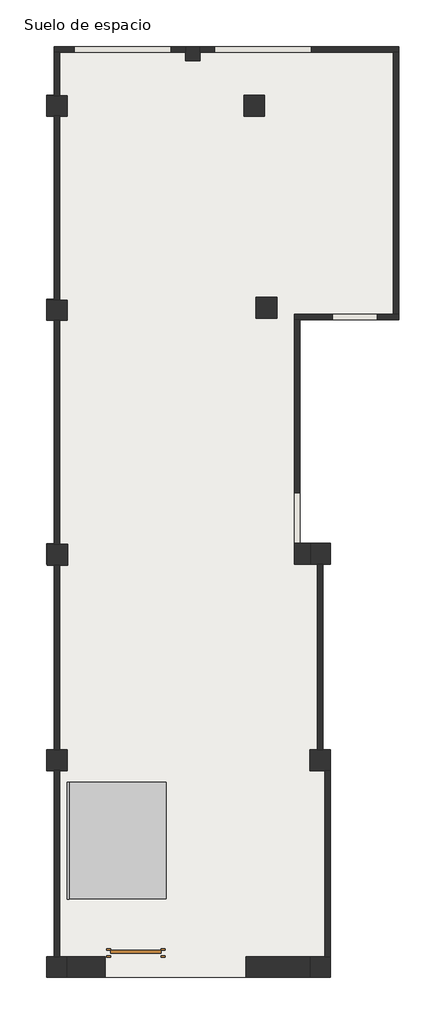
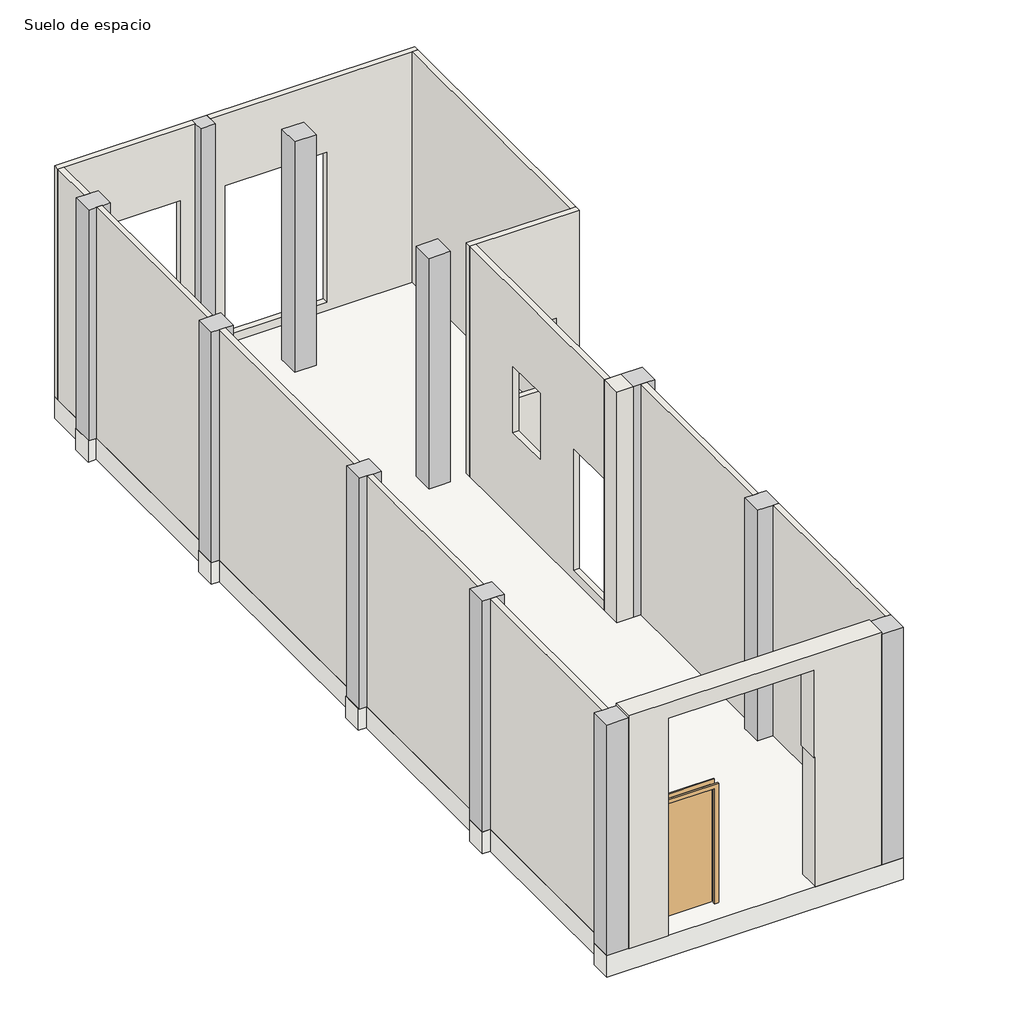
# One storey: 14 walls, 11 columns, 1 door, 1 railing, 1 ramp, 1 slab.
# Revit data of these elements (continued)
# Element 15 (IfcSlab, "Generic Floor - 400mm") (continued)
#   Height Offset From Level = 0.0 cm
#   Phase Created = New Construction
#   Materials on its faces: "Default Roof"
# Elements 16, 17, 18, 19, 20, 21, 22, 23, 24, 25, 26, 27 (IfcWall, "Generic - 100mm Masonry")
#   Top Offset = 0.0 cm
#   Base Offset = 0.0 cm
#   wall height = 426.0 cm
#   Phase Created = Existing
#   Base Constraint = Suelo de espacio
#   Top Constraint = Techo de espacio
#   Materials on its faces: "Concrete, Cast-in-Place gray"
# Element 28 (IfcWall, "Generic - 380mm Masonry")
#   Top Offset = 0.0 cm
#   Base Offset = 0.0 cm
#   wall height = 426.0 cm
#   Phase Created = Existing
#   Base Constraint = Suelo de espacio
#   Top Constraint = Techo de espacio
#   Materials on its faces: "Concrete, Cast-in-Place gray"
# Element 29 (IfcWall, "Generic - 380mm Masonry")
#   Top Offset = 0.0 cm
#   Base Offset = 0.0 cm
#   Unconnected Height = 430.0 cm
#   wall height = 430.0 cm
#   Phase Created = Existing
#   Base Constraint = Suelo de espacio
#   Materials on its faces: "Concrete, Cast-in-Place gray"
# Materials
#   "Door - Panel": class "Wood", colour RGB 114 82 51, transparency 0
#   "Door - Frame": class "Miscellaneous", colour RGB 153 76 43, transparency 0
#   "Concrete, Cast-in-Place gray": class "Concrete", colour RGB 115 116 108, transparency 0, Description = "Cast-in-place concrete", Cost = 0
#   "Default Roof": class "Miscellaneous", colour RGB 80 80 80, transparency 0
